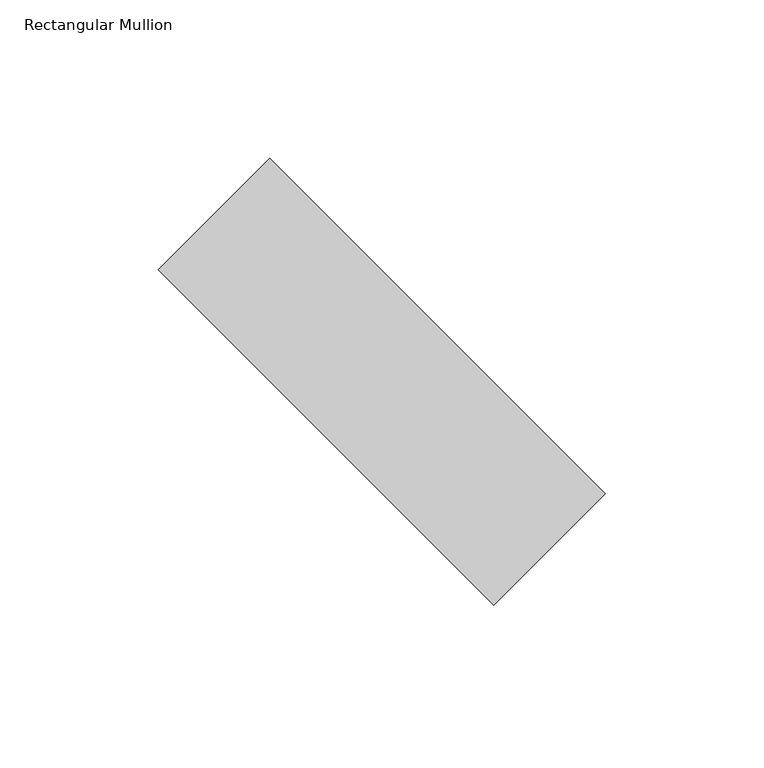
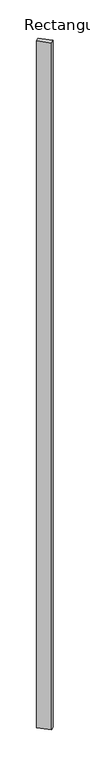
"""IFC4 building model written with IfcOpenShell, lengths in millimetres: member geometry, Rectangular Mullion : tilted mullions."""

from ifc_helpers import new_model, si_unit, frame, origin, place, context, project, spatial, polyline, outline, extrude, source, transform, mapped, element, save


def rectangular_mullion_04c84a83(model_context):
    return source(origin(), model_context, "Body", "SweptSolid", [
        extrude(outline(polyline([(-35.3553391, 70.7106781), (70.7106781, -35.3553391), (35.3553391, -70.7106781), (-70.7106781, 35.3553391), (-35.3553391, 70.7106781)])), frame((0.0, 0.0, -7999.7790849), z_axis=(0.0, 0.0, 1.0), x_axis=(1.0, 0.0, 0.0)), (0.0, 0.0, 1.0), 7999.7790849),
    ])


if __name__ == "__main__":
    model = new_model("IFC4")
    model_context = context("Model", 3, world=origin())
    ifc_project = project(units=[si_unit("LENGTHUNIT", "METRE", prefix="MILLI")], contexts=[model_context])
    site = spatial("IfcSite", under=ifc_project)
    building = spatial("IfcBuilding", under=site)
    placement = place(None, origin())
    rectangular_mullion_shape = rectangular_mullion_04c84a83(model_context)
    element("IfcMember", 1, ObjectType="Rectangular Mullion : tilted mullions", at=placement, inside=building, context=model_context, shape_type="MappedRepresentation", body=[
        mapped(rectangular_mullion_shape, transform((0.0, 0.0, 0.0), x_axis=(1.0, 0.0, 0.0), y_axis=(0.0, 1.0, 0.0), z_axis=(0.0, 0.0, 1.0))),
    ])
    save(model, "model.ifc")

# Revit data of these elements
# Type "Rectangular Mullion : tilted mullions"
#   built-in parameter 1007304 = 0.492126 (stored number, unit not read)
#   built-in parameter 1007301 = 0.082021 (stored number, unit not read)
#   built-in parameter 1007300 = 0.082021 (stored number, unit not read)
# Element 1 (IfcMember, "Rectangular Mullion : tilted mullions")
#   Materials on its faces: "Aluminum"
# Materials
#   "Aluminum": class "Metal", colour RGB 244 244 244, transparency 0, Description = "Aluminum 6061", Cost = 0
